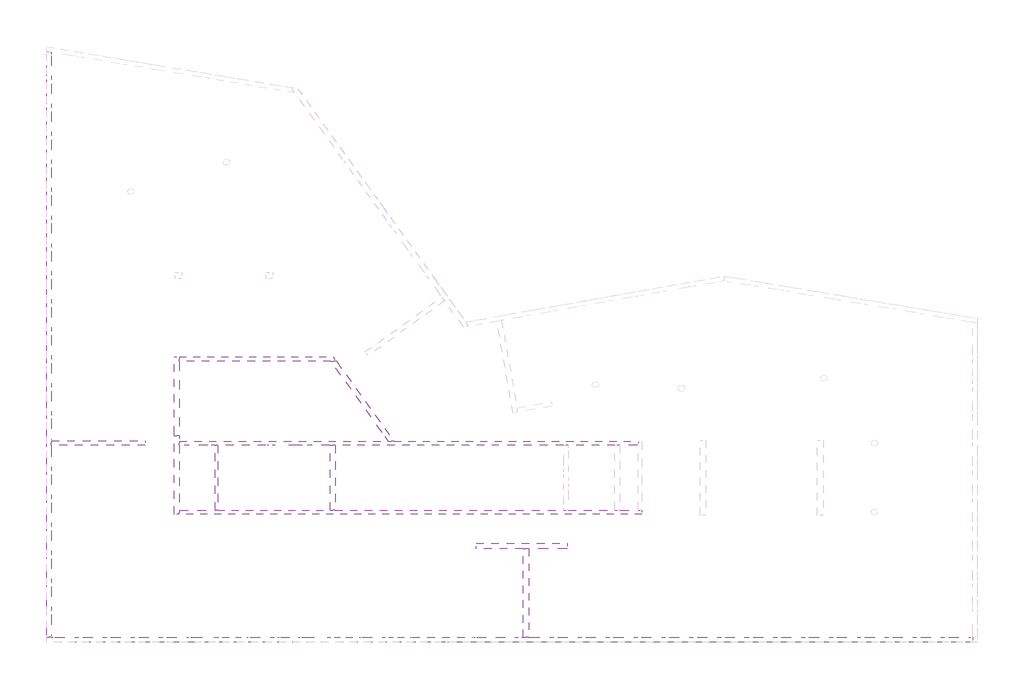
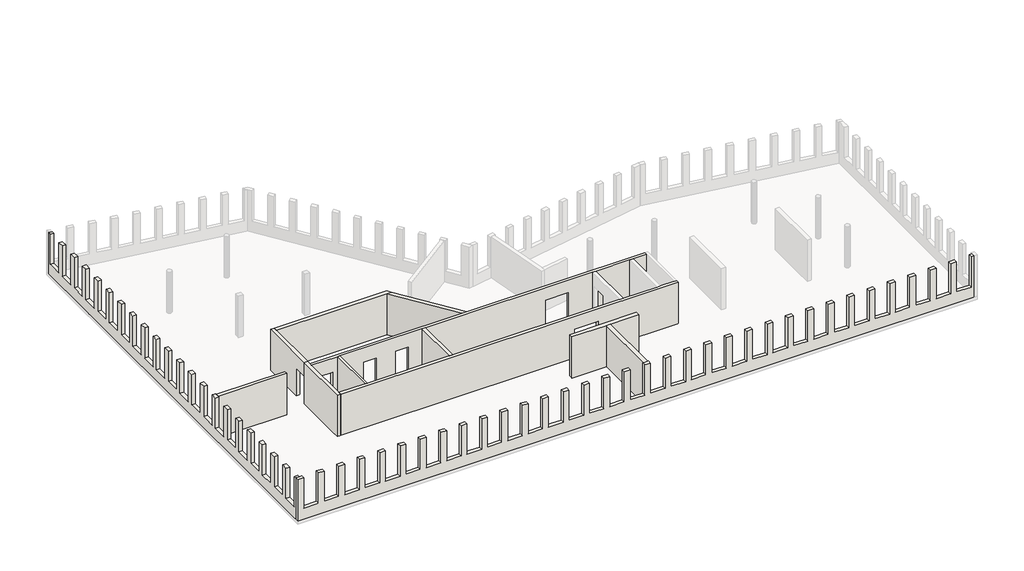
# One storey, part 1 of 2: 13 walls.
"""IFC4 building model written with IfcOpenShell, lengths in millimetres."""

from ifc_helpers import new_model, si_unit, frame, origin, place, context, project, spatial, polyline, outline, extrude, faceted_brep, element, save

model = new_model("IFC4")

# Units and contexts
model_context = context("Model", 3, world=origin())
ifc_project = project(units=[si_unit("LENGTHUNIT", "METRE", prefix="MILLI")], contexts=[model_context])

# Site, building, storey
site = spatial("IfcSite", under=ifc_project)
building = spatial("IfcBuilding", under=site)
storey = spatial("IfcBuildingStorey", under=building, Name="01_OG_OKFB_3,46", Elevation=3460.0)

# Walls
placement = place(None, origin())
element("IfcWall", 1, ObjectType="5dki Lochfassade 26cm C30/37", at=placement, inside=storey, context=model_context, shape_type="Brep", body=[
    faceted_brep([(49396.9999991, 130.0010483, 7630.0), (49396.9999991, 130.0010483, 9980.0), (49603.9991101, 130.0010486, 9980.0), (49603.9991101, 130.0010486, 6770.0), (25766.9999915, 130.0010117, 6770.0), (25466.9999915, 130.0010113, 6770.0), (130.0010047, 130.000972, 6770.0), (-129.9989953, 130.0009716, 6770.0), (-129.9989953, 130.0009716, 9980.0), (130.0010047, 130.000972, 9980.0), (317.0000012, 130.0009723, 9980.0), (316.999997, 130.0009723, 7630.0), (1397.0000012, 130.000974, 7630.0), (1397.0000069, 130.000974, 9980.0), (1816.9999991, 130.0009747, 9980.0), (1817.0000028, 130.0009747, 7630.0), (2896.9999991, 130.0009763, 7630.0), (2897.0000017, 130.0009763, 9980.0), (3316.9999991, 130.000977, 9980.0), (3316.9999977, 130.000977, 7630.0), (4396.9999991, 130.0009787, 7630.0), (4396.9999966, 130.0009787, 9980.0), (4816.9999991, 130.0009793, 9980.0), (4816.9999991, 130.0009793, 7630.0), (5896.9999991, 130.000981, 7630.0), (5896.9999991, 130.000981, 9980.0), (6316.9999991, 130.0009816, 9980.0), (6316.9999991, 130.0009816, 7630.0), (7396.9999991, 130.0009833, 7630.0), (7396.9999991, 130.0009833, 9980.0), (7816.9999991, 130.0009839, 9980.0), (7816.9999991, 130.0009839, 7630.0), (8896.9999991, 130.0009856, 7630.0), (8896.9999991, 130.0009856, 9980.0), (9316.9999991, 130.0009863, 9980.0), (9316.9999991, 130.0009863, 7630.0), (10396.9999991, 130.0009879, 7630.0), (10396.9999991, 130.0009879, 9980.0), (10816.9999991, 130.0009886, 9980.0), (10816.9999991, 130.0009886, 7630.0), (11896.9999991, 130.0009903, 7630.0), (11896.9999991, 130.0009903, 9980.0), (12316.9999991, 130.0009909, 9980.0), (12316.9999991, 130.0009909, 7630.0), (13396.9999991, 130.0009926, 7630.0), (13396.9999991, 130.0009926, 9980.0), (13816.9999991, 130.0009932, 9980.0), (13816.9999991, 130.0009932, 7630.0), (14896.9999991, 130.0009949, 7630.0), (14896.9999991, 130.0009949, 9980.0), (15316.9999991, 130.0009956, 9980.0), (15316.9999991, 130.0009956, 7630.0), (16396.9999991, 130.0009972, 7630.0), (16396.9999991, 130.0009972, 9980.0), (16816.9999991, 130.0009979, 9980.0), (16816.9999991, 130.0009979, 7630.0), (17896.9999991, 130.0009996, 7630.0), (17896.9999991, 130.0009996, 9980.0), (18316.9999991, 130.0010002, 9980.0), (18316.9999991, 130.0010002, 7630.0), (19396.9999991, 130.0010019, 7630.0), (19396.9999991, 130.0010019, 9980.0), (19816.9999991, 130.0010025, 9980.0), (19816.9999991, 130.0010025, 7630.0), (20896.9999991, 130.0010042, 7630.0), (20896.9999991, 130.0010042, 9980.0), (21316.9999991, 130.0010048, 9980.0), (21316.9999991, 130.0010048, 7630.0), (22396.9999991, 130.0010065, 7630.0), (22396.9999991, 130.0010065, 9980.0), (22816.9999991, 130.0010072, 9980.0), (22816.9999991, 130.0010072, 7630.0), (23896.9999991, 130.0010088, 7630.0), (23896.9999991, 130.0010088, 9980.0), (24316.9999991, 130.0010095, 9980.0), (24316.9999991, 130.0010095, 7630.0), (25396.9999991, 130.0010112, 7630.0), (25396.9999991, 130.0010112, 9980.0), (25466.9999915, 130.0010113, 9980.0), (25766.9999915, 130.0010117, 9980.0), (25816.9999991, 130.0010118, 9980.0), (25816.9999991, 130.0010118, 7630.0), (26896.9999991, 130.0010135, 7630.0), (26896.9999991, 130.0010135, 9980.0), (27316.9999991, 130.0010141, 9980.0), (27316.9999991, 130.0010141, 7630.0), (28396.9999991, 130.0010158, 7630.0), (28396.9999991, 130.0010158, 9980.0), (28816.9999991, 130.0010165, 9980.0), (28816.9999991, 130.0010165, 7630.0), (29896.9999991, 130.0010181, 7630.0), (29896.9999991, 130.0010181, 9980.0), (30316.9999991, 130.0010188, 9980.0), (30316.9999991, 130.0010188, 7630.0), (31396.9999991, 130.0010205, 7630.0), (31396.9999991, 130.0010205, 9980.0), (31816.9999991, 130.0010211, 9980.0), (31816.9999991, 130.0010211, 7630.0), (32896.9999991, 130.0010228, 7630.0), (32896.9999991, 130.0010228, 9980.0), (33316.9999991, 130.0010234, 9980.0), (33316.9999991, 130.0010234, 7630.0), (34396.9999991, 130.0010251, 7630.0), (34396.9999991, 130.0010251, 9980.0), (34816.9999991, 130.0010258, 9980.0), (34816.9999991, 130.0010258, 7630.0), (35896.9999991, 130.0010274, 7630.0), (35896.9999991, 130.0010274, 9980.0), (36316.9999991, 130.0010281, 9980.0), (36316.9999991, 130.0010281, 7630.0), (37396.9999991, 130.0010297, 7630.0), (37396.9999991, 130.0010297, 9980.0), (37816.9999991, 130.0010304, 9980.0), (37816.9999991, 130.0010304, 7630.0), (38896.9999991, 130.0010321, 7630.0), (38896.9999991, 130.0010321, 9980.0), (39316.9999991, 130.0010327, 9980.0), (39316.9999991, 130.0010327, 7630.0), (40396.9999991, 130.0010344, 7630.0), (40396.9999991, 130.0010344, 9980.0), (40816.9999991, 130.001035, 9980.0), (40816.9999991, 130.001035, 7630.0), (41896.9999991, 130.0010367, 7630.0), (41896.9999991, 130.0010367, 9980.0), (42316.9999991, 130.0010374, 9980.0), (42316.9999991, 130.0010374, 7630.0), (43396.9999991, 130.001039, 7630.0), (43396.9999991, 130.001039, 9980.0), (43816.9999991, 130.0010397, 9980.0), (43816.9999991, 130.0010397, 7630.0), (44896.9999991, 130.0010414, 7630.0), (44896.9999991, 130.0010414, 9980.0), (45316.9999991, 130.001042, 9980.0), (45316.9999991, 130.001042, 7630.0), (46396.9999991, 130.0010437, 7630.0), (46396.9999991, 130.0010437, 9980.0), (46816.9999991, 130.0010443, 9980.0), (46816.9999991, 130.0010443, 7630.0), (47896.9999991, 130.001046, 7630.0), (47896.9999991, 130.001046, 9980.0), (48316.9999991, 130.0010467, 9980.0), (48316.9999991, 130.0010467, 7630.0), (49603.9991105, -129.9989514, 9980.0), (49396.9999995, -129.9989517, 9980.0), (49396.9999995, -129.9989517, 7630.0), (48316.9999995, -129.9989533, 7630.0), (48316.9999995, -129.9989533, 9980.0), (47896.9999995, -129.998954, 9980.0), (47896.9999995, -129.998954, 7630.0), (46816.9999995, -129.9989557, 7630.0), (46816.9999995, -129.9989557, 9980.0), (46396.9999995, -129.9989563, 9980.0), (46396.9999995, -129.9989563, 7630.0), (45316.9999995, -129.998958, 7630.0), (45316.9999995, -129.998958, 9980.0), (44896.9999995, -129.9989586, 9980.0), (44896.9999995, -129.9989586, 7630.0), (43816.9999995, -129.9989603, 7630.0), (43816.9999995, -129.9989603, 9980.0), (43396.9999995, -129.998961, 9980.0), (43396.9999995, -129.998961, 7630.0), (42316.9999995, -129.9989626, 7630.0), (42316.9999995, -129.9989626, 9980.0), (41896.9999995, -129.9989633, 9980.0), (41896.9999995, -129.9989633, 7630.0), (40816.9999995, -129.998965, 7630.0), (40816.9999995, -129.998965, 9980.0), (40396.9999995, -129.9989656, 9980.0), (40396.9999995, -129.9989656, 7630.0), (39316.9999995, -129.9989673, 7630.0), (39316.9999995, -129.9989673, 9980.0), (38896.9999995, -129.9989679, 9980.0), (38896.9999995, -129.9989679, 7630.0), (37816.9999995, -129.9989696, 7630.0), (37816.9999995, -129.9989696, 9980.0), (37396.9999995, -129.9989703, 9980.0), (37396.9999995, -129.9989703, 7630.0), (36316.9999995, -129.9989719, 7630.0), (36316.9999995, -129.9989719, 9980.0), (35896.9999995, -129.9989726, 9980.0), (35896.9999995, -129.9989726, 7630.0), (34816.9999995, -129.9989742, 7630.0), (34816.9999995, -129.9989742, 9980.0), (34396.9999995, -129.9989749, 9980.0), (34396.9999995, -129.9989749, 7630.0), (33316.9999995, -129.9989766, 7630.0), (33316.9999995, -129.9989766, 9980.0), (32896.9999995, -129.9989772, 9980.0), (32896.9999995, -129.9989772, 7630.0), (31816.9999995, -129.9989789, 7630.0), (31816.9999995, -129.9989789, 9980.0), (31396.9999995, -129.9989795, 9980.0), (31396.9999995, -129.9989795, 7630.0), (30316.9999995, -129.9989812, 7630.0), (30316.9999995, -129.9989812, 9980.0), (29896.9999995, -129.9989819, 9980.0), (29896.9999995, -129.9989819, 7630.0), (28816.9999995, -129.9989835, 7630.0), (28816.9999995, -129.9989835, 9980.0), (28396.9999995, -129.9989842, 9980.0), (28396.9999995, -129.9989842, 7630.0), (27316.9999995, -129.9989859, 7630.0), (27316.9999995, -129.9989859, 9980.0), (26896.9999995, -129.9989865, 9980.0), (26896.9999995, -129.9989865, 7630.0), (25816.9999995, -129.9989882, 7630.0), (25816.9999995, -129.9989882, 9980.0), (25396.9999995, -129.9989888, 9980.0), (25396.9999995, -129.9989888, 7630.0), (24316.9999995, -129.9989905, 7630.0), (24316.9999995, -129.9989905, 9980.0), (23896.9999995, -129.9989912, 9980.0), (23896.9999995, -129.9989912, 7630.0), (22816.9999995, -129.9989928, 7630.0), (22816.9999995, -129.9989928, 9980.0), (22396.9999995, -129.9989935, 9980.0), (22396.9999995, -129.9989935, 7630.0), (21316.9999995, -129.9989952, 7630.0), (21316.9999995, -129.9989952, 9980.0), (20896.9999995, -129.9989958, 9980.0), (20896.9999995, -129.9989958, 7630.0), (19816.9999995, -129.9989975, 7630.0), (19816.9999995, -129.9989975, 9980.0), (19396.9999995, -129.9989981, 9980.0), (19396.9999995, -129.9989981, 7630.0), (18316.9999995, -129.9989998, 7630.0), (18316.9999995, -129.9989998, 9980.0), (17896.9999995, -129.9990004, 9980.0), (17896.9999995, -129.9990004, 7630.0), (16816.9999995, -129.9990021, 7630.0), (16816.9999995, -129.9990021, 9980.0), (16396.9999995, -129.9990028, 9980.0), (16396.9999995, -129.9990028, 7630.0), (15316.9999995, -129.9990044, 7630.0), (15316.9999995, -129.9990044, 9980.0), (14896.9999995, -129.9990051, 9980.0), (14896.9999995, -129.9990051, 7630.0), (13816.9999995, -129.9990068, 7630.0), (13816.9999995, -129.9990068, 9980.0), (13396.9999995, -129.9990074, 9980.0), (13396.9999995, -129.9990074, 7630.0), (12316.9999995, -129.9990091, 7630.0), (12316.9999995, -129.9990091, 9980.0), (11896.9999995, -129.9990097, 9980.0), (11896.9999995, -129.9990097, 7630.0), (10816.9999995, -129.9990114, 7630.0), (10816.9999995, -129.9990114, 9980.0), (10396.9999995, -129.9990121, 9980.0), (10396.9999995, -129.9990121, 7630.0), (9316.9999995, -129.9990137, 7630.0), (9316.9999995, -129.9990137, 9980.0), (8896.9999995, -129.9990144, 9980.0), (8896.9999995, -129.9990144, 7630.0), (7816.9999995, -129.9990161, 7630.0), (7816.9999995, -129.9990161, 9980.0), (7396.9999995, -129.9990167, 9980.0), (7396.9999995, -129.9990167, 7630.0), (6316.9999995, -129.9990184, 7630.0), (6316.9999995, -129.9990184, 9980.0), (5896.9999995, -129.999019, 9980.0), (5896.9999995, -129.999019, 7630.0), (4816.9999995, -129.9990207, 7630.0), (4816.9999995, -129.9990207, 9980.0), (4396.9999995, -129.9990213, 9980.0), (4396.9999966, -129.9990213, 7630.0), (3316.9999995, -129.999023, 7630.0), (3316.9999977, -129.999023, 9980.0), (2896.9999995, -129.9990237, 9980.0), (2897.0000017, -129.9990237, 7630.0), (1816.9999995, -129.9990253, 7630.0), (1817.0000028, -129.9990253, 9980.0), (1397.0000016, -129.999026, 9980.0), (1397.0000069, -129.999026, 7630.0), (317.0000016, -129.9990277, 7630.0), (316.999997, -129.9990277, 9980.0), (-129.9989953, -129.9990284, 9980.0), (-129.9989953, -129.9990284, 6770.0), (49603.9991105, -129.9989514, 6770.0)], [[[0, 1, 2, 3, 4, 5, 6, 7, 8, 9, 10, 11, 12, 13, 14, 15, 16, 17, 18, 19, 20, 21, 22, 23, 24, 25, 26, 27, 28, 29, 30, 31, 32, 33, 34, 35, 36, 37, 38, 39, 40, 41, 42, 43, 44, 45, 46, 47, 48, 49, 50, 51, 52, 53, 54, 55, 56, 57, 58, 59, 60, 61, 62, 63, 64, 65, 66, 67, 68, 69, 70, 71, 72, 73, 74, 75, 76, 77, 78, 79, 80, 81, 82, 83, 84, 85, 86, 87, 88, 89, 90, 91, 92, 93, 94, 95, 96, 97, 98, 99, 100, 101, 102, 103, 104, 105, 106, 107, 108, 109, 110, 111, 112, 113, 114, 115, 116, 117, 118, 119, 120, 121, 122, 123, 124, 125, 126, 127, 128, 129, 130, 131, 132, 133, 134, 135, 136, 137, 138, 139, 140, 141]], [[142, 143, 144, 145, 146, 147, 148, 149, 150, 151, 152, 153, 154, 155, 156, 157, 158, 159, 160, 161, 162, 163, 164, 165, 166, 167, 168, 169, 170, 171, 172, 173, 174, 175, 176, 177, 178, 179, 180, 181, 182, 183, 184, 185, 186, 187, 188, 189, 190, 191, 192, 193, 194, 195, 196, 197, 198, 199, 200, 201, 202, 203, 204, 205, 206, 207, 208, 209, 210, 211, 212, 213, 214, 215, 216, 217, 218, 219, 220, 221, 222, 223, 224, 225, 226, 227, 228, 229, 230, 231, 232, 233, 234, 235, 236, 237, 238, 239, 240, 241, 242, 243, 244, 245, 246, 247, 248, 249, 250, 251, 252, 253, 254, 255, 256, 257, 258, 259, 260, 261, 262, 263, 264, 265, 266, 267, 268, 269, 270, 271, 272, 273, 274, 275, 276, 277]], [[7, 6, 5, 4, 3, 277, 276]], [[17, 267, 266, 18]], [[270, 14, 13, 271]], [[263, 262, 22, 21]], [[259, 258, 26, 25]], [[255, 254, 30, 29]], [[251, 250, 34, 33]], [[247, 246, 38, 37]], [[243, 242, 42, 41]], [[239, 238, 46, 45]], [[235, 234, 50, 49]], [[231, 230, 54, 53]], [[227, 226, 58, 57]], [[223, 222, 62, 61]], [[219, 218, 66, 65]], [[215, 214, 70, 69]], [[211, 210, 74, 73]], [[207, 206, 80, 79, 78, 77]], [[203, 202, 84, 83]], [[199, 198, 88, 87]], [[195, 194, 92, 91]], [[191, 190, 96, 95]], [[187, 186, 100, 99]], [[183, 182, 104, 103]], [[179, 178, 108, 107]], [[175, 174, 112, 111]], [[171, 170, 116, 115]], [[167, 166, 120, 119]], [[163, 162, 124, 123]], [[159, 158, 128, 127]], [[155, 154, 132, 131]], [[151, 150, 136, 135]], [[140, 139, 147, 146]], [[2, 1, 143, 142]], [[10, 9, 8, 275, 274]], [[3, 2, 142, 277]], [[12, 272, 271, 13]], [[273, 11, 10, 274]], [[272, 12, 11, 273]], [[16, 268, 267, 17]], [[269, 15, 14, 270]], [[268, 16, 15, 269]], [[20, 264, 263, 21]], [[265, 19, 18, 266]], [[264, 20, 19, 265]], [[25, 24, 260, 259]], [[23, 22, 262, 261]], [[24, 23, 261, 260]], [[29, 28, 256, 255]], [[27, 26, 258, 257]], [[28, 27, 257, 256]], [[33, 32, 252, 251]], [[31, 30, 254, 253]], [[32, 31, 253, 252]], [[37, 36, 248, 247]], [[35, 34, 250, 249]], [[36, 35, 249, 248]], [[41, 40, 244, 243]], [[39, 38, 246, 245]], [[40, 39, 245, 244]], [[45, 44, 240, 239]], [[43, 42, 242, 241]], [[44, 43, 241, 240]], [[49, 48, 236, 235]], [[47, 46, 238, 237]], [[48, 47, 237, 236]], [[53, 52, 232, 231]], [[51, 50, 234, 233]], [[52, 51, 233, 232]], [[57, 56, 228, 227]], [[55, 54, 230, 229]], [[56, 55, 229, 228]], [[61, 60, 224, 223]], [[59, 58, 226, 225]], [[60, 59, 225, 224]], [[65, 64, 220, 219]], [[63, 62, 222, 221]], [[64, 63, 221, 220]], [[69, 68, 216, 215]], [[67, 66, 218, 217]], [[68, 67, 217, 216]], [[73, 72, 212, 211]], [[71, 70, 214, 213]], [[72, 71, 213, 212]], [[77, 76, 208, 207]], [[75, 74, 210, 209]], [[76, 75, 209, 208]], [[83, 82, 204, 203]], [[81, 80, 206, 205]], [[82, 81, 205, 204]], [[87, 86, 200, 199]], [[85, 84, 202, 201]], [[86, 85, 201, 200]], [[91, 90, 196, 195]], [[89, 88, 198, 197]], [[90, 89, 197, 196]], [[95, 94, 192, 191]], [[93, 92, 194, 193]], [[94, 93, 193, 192]], [[99, 98, 188, 187]], [[97, 96, 190, 189]], [[98, 97, 189, 188]], [[103, 102, 184, 183]], [[101, 100, 186, 185]], [[102, 101, 185, 184]], [[107, 106, 180, 179]], [[105, 104, 182, 181]], [[106, 105, 181, 180]], [[111, 110, 176, 175]], [[109, 108, 178, 177]], [[110, 109, 177, 176]], [[115, 114, 172, 171]], [[113, 112, 174, 173]], [[114, 113, 173, 172]], [[119, 118, 168, 167]], [[117, 116, 170, 169]], [[118, 117, 169, 168]], [[123, 122, 164, 163]], [[121, 120, 166, 165]], [[122, 121, 165, 164]], [[127, 126, 160, 159]], [[125, 124, 162, 161]], [[126, 125, 161, 160]], [[131, 130, 156, 155]], [[129, 128, 158, 157]], [[130, 129, 157, 156]], [[135, 134, 152, 151]], [[133, 132, 154, 153]], [[134, 133, 153, 152]], [[139, 138, 148, 147]], [[137, 136, 150, 149]], [[138, 137, 149, 148]], [[146, 145, 141, 140]], [[144, 143, 1, 0]], [[145, 144, 0, 141]], [[8, 7, 276, 275]]]),
])
element("IfcWall", 2, ObjectType="5dki STB-Wand Kern 25cm C30/37", at=placement, inside=storey, context=model_context, shape_type="Brep", body=[
    faceted_brep([(6989.9999766, 15192.0124447, 9980.0), (6989.9999766, 14942.0124447, 9980.0), (6989.9999766, 10947.0136187, 9980.0), (6989.9999766, 10947.0136187, 8905.0), (6989.9999766, 11957.013616, 8905.0), (6989.9999766, 11957.013616, 6770.0), (6989.9999766, 14942.0124447, 6770.0), (6989.9999766, 15192.0124447, 6770.0), (6739.9999766, 10947.0136187, 9980.0), (6739.9999766, 15192.0124447, 9980.0), (6739.9999766, 15192.0124447, 6770.0), (6739.9999766, 11957.013616, 6770.0), (6739.9999766, 11957.013616, 8905.0), (6739.9999766, 10947.0136187, 8905.0)], [[[0, 1, 2, 3, 4, 5, 6, 7]], [[8, 9, 10, 11, 12, 13]], [[10, 7, 6, 5, 11]], [[2, 1, 0, 9, 8]], [[2, 8, 13, 3]], [[0, 7, 10, 9]], [[4, 12, 11, 5]], [[12, 4, 3, 13]]]),
])
element("IfcWall", 3, ObjectType="5dki STB-Wand Kern 25cm C30/37", at=placement, inside=storey, context=model_context, shape_type="Brep", body=[
    faceted_brep([(6989.9999766, 14942.0124447, 6770.0), (15141.8279932, 14942.0124447, 6770.0), (15449.8792779, 14942.0124447, 6770.0), (15449.8792779, 14942.0124447, 9980.0), (15141.8279932, 14942.0124447, 9980.0), (6989.9999766, 14942.0124447, 9980.0), (6989.9999766, 15192.0124447, 6770.0), (6989.9999766, 15192.0124447, 9980.0), (15269.8915173, 15192.0124447, 9980.0), (15269.8915173, 15192.0124447, 6770.0)], [[[0, 1, 2, 3, 4, 5]], [[6, 7, 8, 9]], [[2, 1, 0, 6, 9]], [[5, 4, 3, 8, 7]], [[0, 5, 7, 6]], [[3, 2, 9, 8]]]),
])
element("IfcWall", 4, ObjectType="5dki STB-Wand Kern 25cm C30/37", at=placement, inside=storey, context=model_context, shape_type="Brep", body=[
    faceted_brep([(18223.2182524, 10662.0127257, 9980.0), (15141.8279932, 14942.0124447, 9980.0), (15141.8279932, 14942.0124447, 6770.0), (17305.3310134, 11936.9428041, 6770.0), (17305.3310134, 11936.9428041, 8905.0), (17895.4523577, 11117.2740911, 8905.0), (17895.4523577, 11117.2740911, 6770.0), (18223.2182524, 10662.0127257, 6770.0), (15449.8792779, 14942.0124447, 9980.0), (18531.2695366, 10662.0127262, 9980.0), (18531.2695366, 10662.0127262, 6770.0), (18098.340653, 11263.3437308, 6770.0), (18098.340653, 11263.3437308, 8905.0), (17508.2193087, 12083.0124438, 8905.0), (17508.2193087, 12083.0124438, 6770.0), (15449.8792779, 14942.0124447, 6770.0)], [[[0, 1, 2, 3, 4, 5, 6, 7]], [[8, 9, 10, 11, 12, 13, 14, 15]], [[2, 15, 14, 3]], [[10, 7, 6, 11]], [[1, 0, 9, 8]], [[2, 1, 8, 15]], [[0, 7, 10, 9]], [[13, 4, 3, 14]], [[4, 13, 12, 5]], [[5, 12, 11, 6]]]),
])
element("IfcWall", 5, ObjectType="5dki STB-Wand Kern 25cm C30/37", at=placement, inside=storey, context=model_context, shape_type="Brep", body=[
    faceted_brep([(6739.9995723, 10947.0136187, 6770.0), (6739.9995723, 6740.0000204, 6770.0), (6739.9995723, 6740.0000204, 9980.0), (6739.9995723, 10947.0136187, 9980.0), (6739.9995723, 10947.0136187, 8905.0), (6989.9995723, 10947.0136187, 6770.0), (6989.9995723, 10947.0136187, 8905.0), (6989.9995723, 10947.0136187, 9980.0), (6989.9995723, 10662.0127052, 9980.0), (6989.9995723, 10442.0127052, 9980.0), (6989.9995723, 6960.0000208, 9980.0), (6989.9995723, 6740.0000208, 9980.0), (6989.9995723, 6740.0000208, 6770.0), (6989.9995723, 6960.0000208, 6770.0), (6989.9995723, 10442.0127052, 6770.0), (6989.9995723, 10662.0127052, 6770.0)], [[[0, 1, 2, 3, 4]], [[5, 6, 7, 8, 9, 10, 11, 12, 13, 14, 15]], [[1, 0, 5, 15, 14, 13, 12]], [[3, 2, 11, 10, 9, 8, 7]], [[0, 4, 3, 7, 6, 5]], [[2, 1, 12, 11]]]),
])
element("IfcWall", 6, ObjectType="5dki STB-Wand Kern 22cm C30/37", at=placement, inside=storey, context=model_context, shape_type="Brep", body=[
    faceted_brep([(31841.999935, 6740.0000516, 9980.0), (6989.9995723, 6740.0000208, 9980.0), (6989.9995723, 6740.0000208, 6770.0), (24166.9999591, 6740.0000421, 6770.0), (24166.999888, 6740.0000421, 9030.0), (25926.9999591, 6740.0000443, 9030.0), (25927.000338, 6740.0000443, 6770.0), (31841.999935, 6740.0000516, 6770.0), (6989.9995723, 6960.0000208, 9980.0), (8916.9999886, 6960.0000232, 9980.0), (9066.9999886, 6960.0000233, 9980.0), (15117.0008797, 6960.0000309, 9980.0), (15367.0008797, 6960.0000312, 9980.0), (27641.9999886, 6960.0000464, 9980.0), (27891.9999886, 6960.0000467, 9980.0), (30391.9999891, 6960.0000498, 9980.0), (30641.9999891, 6960.0000501, 9980.0), (31641.9999382, 6960.0000514, 9980.0), (31841.9999382, 6960.0000516, 9980.0), (31841.9999382, 6960.0000516, 6770.0), (31641.9999382, 6960.0000514, 6770.0), (30641.9999891, 6960.0000501, 6770.0), (30391.9999891, 6960.0000498, 6770.0), (27891.9999886, 6960.0000467, 6770.0), (27641.9999886, 6960.0000464, 6770.0), (25926.9999588, 6960.0000443, 6770.0), (25927.000338, 6960.0000443, 9030.0), (24166.9999588, 6960.0000421, 9030.0), (24166.999888, 6960.0000421, 6770.0), (15367.0008797, 6960.0000312, 6770.0), (15117.0008797, 6960.0000309, 6770.0), (9066.9999886, 6960.0000233, 6770.0), (8916.9999886, 6960.0000232, 6770.0), (6989.9995723, 6960.0000208, 6770.0)], [[[0, 1, 2, 3, 4, 5, 6, 7]], [[8, 9, 10, 11, 12, 13, 14, 15, 16, 17, 18, 19, 20, 21, 22, 23, 24, 25, 26, 27, 28, 29, 30, 31, 32, 33]], [[2, 33, 32, 31, 30, 29, 28, 3]], [[19, 7, 6, 25, 24, 23, 22, 21, 20]], [[1, 0, 18, 17, 16, 15, 14, 13, 12, 11, 10, 9, 8]], [[2, 1, 8, 33]], [[0, 7, 19, 18]], [[5, 26, 25, 6]], [[26, 5, 4, 27]], [[27, 4, 3, 28]]]),
])
element("IfcWall", 7, ObjectType="5dki STB-Wand Kern 22cm C30/37", at=placement, inside=storey, context=model_context, shape_type="Brep", body=[
    faceted_brep([(6989.9995723, 10662.0127052, 9980.0), (18223.2182524, 10662.0127257, 9980.0), (18531.2695366, 10662.0127262, 9980.0), (31641.9999912, 10662.0127502, 9980.0), (31641.9999912, 10662.0127502, 6770.0), (25926.999945, 10662.0127397, 6770.0), (25927.0000254, 10662.0127397, 9030.0), (24166.999945, 10662.0127365, 9030.0), (24166.9998144, 10662.0127365, 6770.0), (18531.2695366, 10662.0127262, 6770.0), (18223.2182524, 10662.0127257, 6770.0), (14152.0004935, 10662.0127182, 6770.0), (14152.0007698, 10662.0127182, 8905.0), (13142.0004935, 10662.0127164, 8905.0), (13142.0009721, 10662.0127164, 6770.0), (11796.9999806, 10662.0127139, 6770.0), (11796.9997327, 10662.0127139, 8905.0), (10786.9999806, 10662.0127121, 8905.0), (10786.999935, 10662.0127121, 6770.0), (8540.0010342, 10662.012708, 6770.0), (8540.000485, 10662.012708, 8905.0), (7530.0010342, 10662.0127061, 8905.0), (7530.0006873, 10662.0127061, 6770.0), (6989.9995723, 10662.0127052, 6770.0), (31641.9999881, 10442.0127502, 9980.0), (30641.9999891, 10442.0127483, 9980.0), (30391.9999891, 10442.0127479, 9980.0), (27891.9999829, 10442.0127433, 9980.0), (27641.9999829, 10442.0127429, 9980.0), (15367.0008797, 10442.0127204, 9980.0), (15117.0008797, 10442.01272, 9980.0), (9066.9999886, 10442.0127089, 9980.0), (8916.9999886, 10442.0127087, 9980.0), (6989.9995723, 10442.0127052, 9980.0), (6989.9995723, 10442.0127052, 6770.0), (7530.0010346, 10442.0127061, 6770.0), (7530.0006873, 10442.0127061, 8905.0), (8540.0010346, 10442.012708, 8905.0), (8540.000485, 10442.012708, 6770.0), (8916.9999886, 10442.0127087, 6770.0), (9066.9999886, 10442.0127089, 6770.0), (10786.999981, 10442.0127121, 6770.0), (10786.999935, 10442.0127121, 8905.0), (11796.999981, 10442.0127139, 8905.0), (11796.9997327, 10442.0127139, 6770.0), (13142.0004939, 10442.0127164, 6770.0), (13142.0009721, 10442.0127164, 8905.0), (14152.0004939, 10442.0127182, 8905.0), (14152.0007698, 10442.0127182, 6770.0), (15117.0008797, 10442.01272, 6770.0), (15367.0008797, 10442.0127204, 6770.0), (24166.9999454, 10442.0127365, 6770.0), (24166.9998144, 10442.0127365, 9030.0), (25926.9999454, 10442.0127397, 9030.0), (25927.0000254, 10442.0127397, 6770.0), (27641.9999829, 10442.0127429, 6770.0), (27891.9999829, 10442.0127433, 6770.0), (30391.9999891, 10442.0127479, 6770.0), (30641.9999891, 10442.0127483, 6770.0), (31641.9999881, 10442.0127502, 6770.0)], [[[0, 1, 2, 3, 4, 5, 6, 7, 8, 9, 10, 11, 12, 13, 14, 15, 16, 17, 18, 19, 20, 21, 22, 23]], [[24, 25, 26, 27, 28, 29, 30, 31, 32, 33, 34, 35, 36, 37, 38, 39, 40, 41, 42, 43, 44, 45, 46, 47, 48, 49, 50, 51, 52, 53, 54, 55, 56, 57, 58, 59]], [[34, 23, 22, 35]], [[4, 59, 58, 57, 56, 55, 54, 5]], [[8, 51, 50, 49, 48, 11, 10, 9]], [[18, 41, 40, 39, 38, 19]], [[44, 15, 14, 45]], [[3, 2, 1, 0, 33, 32, 31, 30, 29, 28, 27, 26, 25, 24]], [[0, 23, 34, 33]], [[4, 3, 24, 59]], [[53, 6, 5, 54]], [[6, 53, 52, 7]], [[7, 52, 51, 8]], [[17, 42, 41, 18]], [[42, 17, 16, 43]], [[43, 16, 15, 44]], [[13, 46, 45, 14]], [[46, 13, 12, 47]], [[47, 12, 11, 48]], [[21, 36, 35, 22]], [[36, 21, 20, 37]], [[37, 20, 19, 38]]]),
])
element("IfcWall", 8, ObjectType="5dki STB-Wand Kern 25cm C30/37", at=placement, inside=storey, context=model_context, shape_type="SweptSolid", body=[
    extrude(outline(polyline([(15117.0008797, 6960.0000309), (15117.0008797, 10442.01272), (15367.0008797, 10442.0127204), (15367.0008797, 6960.0000312), (15117.0008797, 6960.0000309)])), frame((0.0, 0.0, 6770.0), z_axis=(0.0, 0.0, 1.0), x_axis=(1.0, 0.0, 0.0)), (0.0, 0.0, 1.0), 3210.0),
])
element("IfcWall", 9, ObjectType="5dki STB-Wand Kern 15cm C30/37", at=placement, inside=storey, context=model_context, shape_type="SweptSolid", body=[
    extrude(outline(polyline([(8916.9999886, 6960.0000232), (8916.9999886, 10442.0127087), (9066.9999886, 10442.0127089), (9066.9999886, 6960.0000233), (8916.9999886, 6960.0000232)])), frame((0.0, 0.0, 6770.0), z_axis=(0.0, 0.0, 1.0), x_axis=(1.0, 0.0, 0.0)), (0.0, 0.0, 1.0), 3210.0),
])
element("IfcWall", 10, ObjectType="5dki Lochfassade 26cm C30/37", at=placement, inside=storey, context=model_context, shape_type="Brep", body=[
    faceted_brep([(130.0010047, 24278.4322867, 7630.0), (130.0010047, 24278.4322867, 9980.0), (130.0010047, 23857.0124158, 9980.0), (130.0010047, 23857.0124158, 7630.0), (130.0010047, 22777.0124158, 7630.0), (130.0010047, 22777.0124158, 9980.0), (130.0010047, 22357.0124158, 9980.0), (130.0010047, 22357.0124158, 7630.0), (130.0010047, 21277.0124158, 7630.0), (130.0010047, 21277.0124158, 9980.0), (130.0010047, 20857.0124158, 9980.0), (130.0010047, 20857.0124158, 7630.0), (130.0010047, 19777.0124158, 7630.0), (130.0010047, 19777.0124158, 9980.0), (130.0010047, 19357.0124158, 9980.0), (130.0010047, 19357.0124158, 7630.0), (130.0010047, 18277.0124158, 7630.0), (130.0010047, 18277.0124158, 9980.0), (130.0010047, 17857.0124158, 9980.0), (130.0010047, 17857.0124158, 7630.0), (130.0010047, 16777.0124158, 7630.0), (130.0010047, 16777.0124158, 9980.0), (130.0010047, 16357.0124158, 9980.0), (130.0010047, 16357.0124158, 7630.0), (130.0010047, 15277.0124158, 7630.0), (130.0010047, 15277.0124158, 9980.0), (130.0010047, 14857.0124158, 9980.0), (130.0010047, 14857.0124158, 7630.0), (130.0010047, 13777.0124158, 7630.0), (130.0010047, 13777.0124158, 9980.0), (130.0010047, 13357.0124158, 9980.0), (130.0010047, 13357.0124158, 7630.0), (130.0010047, 12277.0124158, 7630.0), (130.0010047, 12277.0124158, 9980.0), (130.0010047, 11857.0124158, 9980.0), (130.0010047, 11857.0124158, 7630.0), (130.0010047, 10777.0124158, 7630.0), (130.0010047, 10777.0124158, 9980.0), (130.0010047, 10692.0124295, 9980.0), (130.0010047, 10442.0124295, 9980.0), (130.0010047, 10357.0124158, 9980.0), (130.0010047, 10357.0124158, 7630.0), (130.0010047, 9277.0124158, 7630.0), (130.0010047, 9277.0124158, 9980.0), (130.0010047, 8857.0124158, 9980.0), (130.0010047, 8857.0124158, 7630.0), (130.0010047, 7777.0124158, 7630.0), (130.0010047, 7777.0124158, 9980.0), (130.0010047, 7357.0124158, 9980.0), (130.0010047, 7357.0124158, 7630.0), (130.0010047, 6277.0124158, 7630.0), (130.0010047, 6277.0124158, 9980.0), (130.0010047, 5857.0124158, 9980.0), (130.0010047, 5857.0124158, 7630.0), (130.0010047, 4777.0124158, 7630.0), (130.0010047, 4777.0124158, 9980.0), (130.0010047, 4357.0124158, 9980.0), (130.0010047, 4357.0124158, 7630.0), (130.0010047, 3277.0124158, 7630.0), (130.0010047, 3277.0124158, 9980.0), (130.0010047, 2857.0124158, 9980.0), (130.0010047, 2857.0124158, 7630.0), (130.0010047, 1777.0124158, 7630.0), (130.0010047, 1777.0124158, 9980.0), (130.0010047, 1357.0124158, 9980.0), (130.0010047, 1357.0124158, 7630.0), (130.0010047, 277.0124158, 7630.0), (130.0010047, 277.0124158, 9980.0), (130.0010047, 130.000972, 9980.0), (130.0010047, 130.000972, 6770.0), (130.0010047, 10442.0124295, 6770.0), (130.0010047, 10692.0124295, 6770.0), (130.0010047, 31548.6978518, 6770.0), (130.0010047, 31548.6978518, 9980.0), (130.0010047, 31357.0124158, 9980.0), (130.0010047, 31357.0124158, 7630.0), (130.0010047, 30277.0124158, 7630.0), (130.0010047, 30277.0124158, 9980.0), (130.0010047, 29857.0124158, 9980.0), (130.0010047, 29857.0124158, 7630.0), (130.0010047, 28777.0124158, 7630.0), (130.0010047, 28777.0124158, 9980.0), (130.0010047, 28358.4322867, 9980.0), (130.0010047, 28358.4322867, 7630.0), (130.0010047, 27278.4322867, 7630.0), (130.0010047, 27278.4322867, 9980.0), (130.0010047, 26858.4322867, 9980.0), (130.0010047, 26858.4322867, 7630.0), (130.0010047, 25778.4322867, 7630.0), (130.0010047, 25778.4322867, 9980.0), (130.0010047, 25358.4322867, 9980.0), (130.0010047, 25358.4322867, 7630.0), (-129.9989953, 23857.0124158, 9980.0), (-129.9989953, 24278.4322867, 9980.0), (-129.9989953, 24278.4322867, 7630.0), (-129.9989953, 25358.4322867, 7630.0), (-129.9989953, 25358.4322867, 9980.0), (-129.9989953, 25778.4322867, 9980.0), (-129.9989953, 25778.4322867, 7630.0), (-129.9989953, 26858.4322867, 7630.0), (-129.9989953, 26858.4322867, 9980.0), (-129.9989953, 27278.4322867, 9980.0), (-129.9989953, 27278.4322867, 7630.0), (-129.9989953, 28358.4322867, 7630.0), (-129.9989953, 28358.4322867, 9980.0), (-129.9989953, 28777.0124158, 9980.0), (-129.9989953, 28777.0124158, 7630.0), (-129.9989953, 29857.0124158, 7630.0), (-129.9989953, 29857.0124158, 9980.0), (-129.9989953, 30277.0124158, 9980.0), (-129.9989953, 30277.0124158, 7630.0), (-129.9989953, 31357.0124158, 7630.0), (-129.9989953, 31357.0124158, 9980.0), (-129.9989953, 31592.114918, 9980.0), (-129.9989953, 31592.114918, 6770.0), (-129.9989953, 130.0009716, 6770.0), (-129.9989953, 130.0009716, 9980.0), (-129.9989953, 277.0124158, 9980.0), (-129.9989953, 277.0124158, 7630.0), (-129.9989953, 1357.0124158, 7630.0), (-129.9989953, 1357.0124158, 9980.0), (-129.9989953, 1777.0124158, 9980.0), (-129.9989953, 1777.0124158, 7630.0), (-129.9989953, 2857.0124158, 7630.0), (-129.9989953, 2857.0124158, 9980.0), (-129.9989953, 3277.0124158, 9980.0), (-129.9989953, 3277.0124158, 7630.0), (-129.9989953, 4357.0124158, 7630.0), (-129.9989953, 4357.0124158, 9980.0), (-129.9989953, 4777.0124158, 9980.0), (-129.9989953, 4777.0124158, 7630.0), (-129.9989953, 5857.0124158, 7630.0), (-129.9989953, 5857.0124158, 9980.0), (-129.9989953, 6277.0124158, 9980.0), (-129.9989953, 6277.0124158, 7630.0), (-129.9989953, 7357.0124158, 7630.0), (-129.9989953, 7357.0124158, 9980.0), (-129.9989953, 7777.0124158, 9980.0), (-129.9989953, 7777.0124158, 7630.0), (-129.9989953, 8857.0124158, 7630.0), (-129.9989953, 8857.0124158, 9980.0), (-129.9989953, 9277.0124158, 9980.0), (-129.9989953, 9277.0124158, 7630.0), (-129.9989953, 10357.0124158, 7630.0), (-129.9989953, 10357.0124158, 9980.0), (-129.9989953, 10777.0124158, 9980.0), (-129.9989953, 10777.0124158, 7630.0), (-129.9989953, 11857.0124158, 7630.0), (-129.9989953, 11857.0124158, 9980.0), (-129.9989953, 12277.0124158, 9980.0), (-129.9989953, 12277.0124158, 7630.0), (-129.9989953, 13357.0124158, 7630.0), (-129.9989953, 13357.0124158, 9980.0), (-129.9989953, 13777.0124158, 9980.0), (-129.9989953, 13777.0124158, 7630.0), (-129.9989953, 14857.0124158, 7630.0), (-129.9989953, 14857.0124158, 9980.0), (-129.9989953, 15277.0124158, 9980.0), (-129.9989953, 15277.0124158, 7630.0), (-129.9989953, 16357.0124158, 7630.0), (-129.9989953, 16357.0124158, 9980.0), (-129.9989953, 16777.0124158, 9980.0), (-129.9989953, 16777.0124158, 7630.0), (-129.9989953, 17857.0124158, 7630.0), (-129.9989953, 17857.0124158, 9980.0), (-129.9989953, 18277.0124158, 9980.0), (-129.9989953, 18277.0124158, 7630.0), (-129.9989953, 19357.0124158, 7630.0), (-129.9989953, 19357.0124158, 9980.0), (-129.9989953, 19777.0124158, 9980.0), (-129.9989953, 19777.0124158, 7630.0), (-129.9989953, 20857.0124158, 7630.0), (-129.9989953, 20857.0124158, 9980.0), (-129.9989953, 21277.0124158, 9980.0), (-129.9989953, 21277.0124158, 7630.0), (-129.9989953, 22357.0124158, 7630.0), (-129.9989953, 22357.0124158, 9980.0), (-129.9989953, 22777.0124158, 9980.0), (-129.9989953, 22777.0124158, 7630.0), (-129.9989953, 23857.0124158, 7630.0), (90.4211678, 31555.307238, 9980.0)], [[[0, 1, 2, 3, 4, 5, 6, 7, 8, 9, 10, 11, 12, 13, 14, 15, 16, 17, 18, 19, 20, 21, 22, 23, 24, 25, 26, 27, 28, 29, 30, 31, 32, 33, 34, 35, 36, 37, 38, 39, 40, 41, 42, 43, 44, 45, 46, 47, 48, 49, 50, 51, 52, 53, 54, 55, 56, 57, 58, 59, 60, 61, 62, 63, 64, 65, 66, 67, 68, 69, 70, 71, 72, 73, 74, 75, 76, 77, 78, 79, 80, 81, 82, 83, 84, 85, 86, 87, 88, 89, 90, 91]], [[92, 93, 94, 95, 96, 97, 98, 99, 100, 101, 102, 103, 104, 105, 106, 107, 108, 109, 110, 111, 112, 113, 114, 115, 116, 117, 118, 119, 120, 121, 122, 123, 124, 125, 126, 127, 128, 129, 130, 131, 132, 133, 134, 135, 136, 137, 138, 139, 140, 141, 142, 143, 144, 145, 146, 147, 148, 149, 150, 151, 152, 153, 154, 155, 156, 157, 158, 159, 160, 161, 162, 163, 164, 165, 166, 167, 168, 169, 170, 171, 172, 173, 174, 175, 176, 177, 178, 179]], [[72, 71, 70, 69, 115, 114]], [[64, 63, 121, 120]], [[60, 59, 125, 124]], [[56, 55, 129, 128]], [[52, 51, 133, 132]], [[48, 47, 137, 136]], [[44, 43, 141, 140]], [[40, 39, 38, 37, 145, 144]], [[34, 33, 149, 148]], [[30, 29, 153, 152]], [[26, 25, 157, 156]], [[22, 21, 161, 160]], [[18, 17, 165, 164]], [[14, 13, 169, 168]], [[10, 9, 173, 172]], [[6, 5, 177, 176]], [[74, 73, 180, 113, 112]], [[78, 77, 109, 108]], [[82, 81, 105, 104]], [[86, 85, 101, 100]], [[90, 89, 97, 96]], [[2, 1, 93, 92]], [[116, 68, 67, 117]], [[119, 65, 64, 120]], [[66, 118, 117, 67]], [[65, 119, 118, 66]], [[124, 123, 61, 60]], [[122, 121, 63, 62]], [[123, 122, 62, 61]], [[128, 127, 57, 56]], [[126, 125, 59, 58]], [[127, 126, 58, 57]], [[132, 131, 53, 52]], [[130, 129, 55, 54]], [[131, 130, 54, 53]], [[136, 135, 49, 48]], [[134, 133, 51, 50]], [[135, 134, 50, 49]], [[140, 139, 45, 44]], [[138, 137, 47, 46]], [[139, 138, 46, 45]], [[144, 143, 41, 40]], [[142, 141, 43, 42]], [[143, 142, 42, 41]], [[148, 147, 35, 34]], [[146, 145, 37, 36]], [[147, 146, 36, 35]], [[152, 151, 31, 30]], [[150, 149, 33, 32]], [[151, 150, 32, 31]], [[156, 155, 27, 26]], [[154, 153, 29, 28]], [[155, 154, 28, 27]], [[160, 159, 23, 22]], [[158, 157, 25, 24]], [[159, 158, 24, 23]], [[164, 163, 19, 18]], [[162, 161, 21, 20]], [[163, 162, 20, 19]], [[168, 167, 15, 14]], [[166, 165, 17, 16]], [[167, 166, 16, 15]], [[172, 171, 11, 10]], [[170, 169, 13, 12]], [[171, 170, 12, 11]], [[176, 175, 7, 6]], [[174, 173, 9, 8]], [[175, 174, 8, 7]], [[92, 179, 3, 2]], [[178, 177, 5, 4]], [[179, 178, 4, 3]], [[112, 111, 75, 74]], [[110, 109, 77, 76]], [[111, 110, 76, 75]], [[108, 107, 79, 78]], [[106, 105, 81, 80]], [[107, 106, 80, 79]], [[104, 103, 83, 82]], [[102, 101, 85, 84]], [[103, 102, 84, 83]], [[100, 99, 87, 86]], [[98, 97, 89, 88]], [[99, 98, 88, 87]], [[96, 95, 91, 90]], [[94, 93, 1, 0]], [[95, 94, 0, 91]], [[69, 68, 116, 115]], [[73, 72, 114, 113, 180]]]),
])
element("IfcWall", 11, ObjectType="5dki STB-Wand 25cm C30/37", at=placement, inside=storey, context=model_context, shape_type="SweptSolid", body=[
    extrude(outline(polyline([(130.0010047, 10692.0124295), (5179.9999831, 10692.0124295), (5179.9999831, 10442.0124295), (130.0010047, 10442.0124295), (130.0010047, 10692.0124295)])), frame((0.0, 0.0, 6770.0), z_axis=(0.0, 0.0, 1.0), x_axis=(1.0, 0.0, 0.0)), (0.0, 0.0, 1.0), 3210.0),
])
element("IfcWall", 12, ObjectType="5dki STB-Wand 30cm C30/37", at=placement, inside=storey, context=model_context, shape_type="Brep", body=[
    faceted_brep([(22936.4905033, 4880.0000432, 6770.0), (25466.9999915, 4880.0000432, 6770.0), (25766.9999915, 4880.0000432, 6770.0), (27842.0010332, 4880.0000432, 6770.0), (27842.0010332, 4880.0000432, 9980.0), (25766.9999915, 4880.0000432, 9980.0), (25466.9999915, 4880.0000432, 9980.0), (22936.4905033, 4880.0000432, 9980.0), (22936.4905033, 5180.0000432, 6770.0), (22936.4905033, 5180.0000432, 9980.0), (27842.0010332, 5180.0000432, 9980.0), (27842.0010332, 5180.0000432, 6770.0)], [[[0, 1, 2, 3, 4, 5, 6, 7]], [[8, 9, 10, 11]], [[3, 2, 1, 0, 8, 11]], [[4, 3, 11, 10]], [[7, 6, 5, 4, 10, 9]], [[0, 7, 9, 8]]]),
])
element("IfcWall", 13, ObjectType="5dki STB-Wand 30cm C30/37", at=placement, inside=storey, context=model_context, shape_type="SweptSolid", body=[
    extrude(outline(polyline([(25466.9999915, 130.0010113), (25466.9999915, 4880.0000432), (25766.9999915, 4880.0000432), (25766.9999915, 130.0010117), (25466.9999915, 130.0010113)])), frame((0.0, 0.0, 6770.0), z_axis=(0.0, 0.0, 1.0), x_axis=(1.0, 0.0, 0.0)), (0.0, 0.0, 1.0), 3210.0),
])

save(model, "model.ifc")

# Revit data of these elements
# Type "5dki Lochfassade 26cm C30/37"
#   Type Comments = ""
#   Description = ""
#   cpiComponentType = "Wall"
#   cpiFitMatchKey = "5D-KI-STB-OB-W-LF"
#   5d Materialgüte = "C35/45"
#   Filter Tragend / Nichttragend = yes
#   5dki WU = no
#   Layers, outside or top first: 0.260 m "5d Beton - Stahlbeton" (function 1)
# Type "5dki STB-Wand Kern 25cm C30/37"
#   Type Comments = ""
#   Description = ""
#   cpiComponentType = "Wall"
#   cpiFitMatchKey = "5D-KI-STB-OB-W-K"
#   5d Materialgüte = "C30/37"
#   Filter Tragend / Nichttragend = yes
#   5dki WU = no
#   Layers, outside or top first: 0.250 m "5d Beton - Stahlbeton" (function 1)
# Type "5dki STB-Wand Kern 22cm C30/37"
#   Type Comments = ""
#   Description = ""
#   cpiComponentType = "Wall"
#   cpiFitMatchKey = "5D-KI-STB-OB-W-K"
#   5d Materialgüte = "C30/37"
#   Filter Tragend / Nichttragend = yes
#   5dki WU = no
#   Layers, outside or top first: 0.220 m "5d Beton - Stahlbeton" (function 1)
# Type "5dki STB-Wand Kern 15cm C30/37"
#   Type Comments = ""
#   Description = ""
#   cpiComponentType = "Wall"
#   cpiFitMatchKey = "5D-KI-STB-OB-W-K"
#   5d Materialgüte = "C30/37"
#   Filter Tragend / Nichttragend = yes
#   5dki WU = no
#   Layers, outside or top first: 0.150 m "5d Beton - Stahlbeton" (function 1)
# Type "5dki STB-Wand 25cm C30/37"
#   Type Comments = ""
#   Description = ""
#   cpiComponentType = "Wall"
#   cpiFitMatchKey = "5D-KI-STB-OB-W"
#   5d Materialgüte = "C30/37"
#   Filter Tragend / Nichttragend = yes
#   5dki WU = no
#   Layers, outside or top first: 0.250 m "5d Beton - Stahlbeton" (function 1)
# Type "5dki STB-Wand 30cm C30/37"
#   Type Comments = ""
#   Description = ""
#   cpiComponentType = "Wall"
#   cpiFitMatchKey = "5D-KI-STB-OB-W"
#   5d Materialgüte = "C30/37"
#   Filter Tragend / Nichttragend = yes
#   5dki WU = no
#   Layers, outside or top first: 0.300 m "5d Beton - Stahlbeton" (function 1)
# Element 1 (IfcWall, "5dki Lochfassade 26cm C30/37")
#   000_080_030_Geschoß = "02_OG"
#   Top Offset = 0.000 m
#   Base Offset = 0.000 m
#   wall height = 3.210 m
#   Phase Created = Neu
#   Base Constraint = 01_OG_OKRD_6,77
#   Top Constraint = 02_OG_UKRD_9,98
#   Materials on its faces: "5d Beton - Stahlbeton"
# Elements 2, 3, 4, 5, 8 (IfcWall, "5dki STB-Wand Kern 25cm C30/37")
#   Comments = ""
#   000_080_030_Geschoß = "02_OG"
#   Top Offset = 0.000 m
#   Base Offset = 0.000 m
#   wall height = 3.210 m
#   Phase Created = Neu
#   Base Constraint = 01_OG_OKRD_6,77
#   Top Constraint = 02_OG_UKRD_9,98
#   Materials on its faces: "5d Beton - Stahlbeton"
# Elements 6, 7 (IfcWall, "5dki STB-Wand Kern 22cm C30/37")
#   Comments = ""
#   000_080_030_Geschoß = "02_OG"
#   Top Offset = 0.000 m
#   Base Offset = 0.000 m
#   wall height = 3.210 m
#   Phase Created = Neu
#   Base Constraint = 01_OG_OKRD_6,77
#   Top Constraint = 02_OG_UKRD_9,98
#   Materials on its faces: "5d Beton - Stahlbeton"
# Element 9 (IfcWall, "5dki STB-Wand Kern 15cm C30/37")
#   Comments = ""
#   000_080_030_Geschoß = "02_OG"
#   Top Offset = 0.000 m
#   Base Offset = 0.000 m
#   wall height = 3.210 m
#   Phase Created = Neu
#   Base Constraint = 01_OG_OKRD_6,77
#   Top Constraint = 02_OG_UKRD_9,98
#   Materials on its faces: "5d Beton - Stahlbeton"
# Element 10 (IfcWall, "5dki Lochfassade 26cm C30/37")
#   Comments = ""
#   000_080_030_Geschoß = "02_OG"
#   Top Offset = 0.000 m
#   Base Offset = 0.000 m
#   wall height = 3.210 m
#   Phase Created = Neu
#   Base Constraint = 01_OG_OKRD_6,77
#   Top Constraint = 02_OG_UKRD_9,98
#   Materials on its faces: "5d Beton - Stahlbeton"
# Element 11 (IfcWall, "5dki STB-Wand 25cm C30/37")
#   Comments = ""
#   000_080_030_Geschoß = "02_OG"
#   Top Offset = 0.000 m
#   Base Offset = 0.000 m
#   wall height = 3.210 m
#   Phase Created = Neu
#   Base Constraint = 01_OG_OKRD_6,77
#   Top Constraint = 02_OG_UKRD_9,98
#   Materials on its faces: "5d Beton - Stahlbeton"
# Element 12 (IfcWall, "5dki STB-Wand 30cm C30/37")
#   Comments = ""
#   000_080_030_Geschoß = "02_OG"
#   Top Offset = 0.000 m
#   Base Offset = 0.000 m
#   wall height = 3.210 m
#   Phase Created = Neu
#   Base Constraint = 01_OG_OKRD_6,77
#   Top Constraint = 02_OG_UKRD_9,98
#   Materials on its faces: "5d Beton - Stahlbeton"
# Element 13 (IfcWall, "5dki STB-Wand 30cm C30/37")
#   000_080_030_Geschoß = "02_OG"
#   Top Offset = 0.000 m
#   Base Offset = 0.000 m
#   wall height = 3.210 m
#   Phase Created = Neu
#   Base Constraint = 01_OG_OKRD_6,77
#   Top Constraint = 02_OG_UKRD_9,98
#   Materials on its faces: "5d Beton - Stahlbeton"
# Materials
#   "5d Beton - Stahlbeton": class "5dki", colour RGB 200 200 200, transparency 0, Cost = 0
